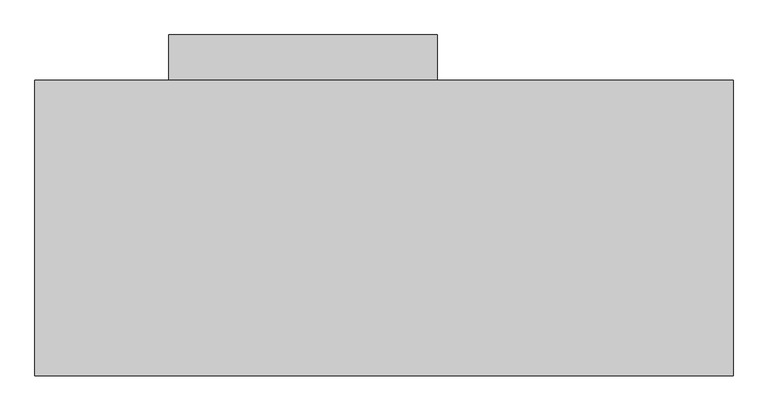
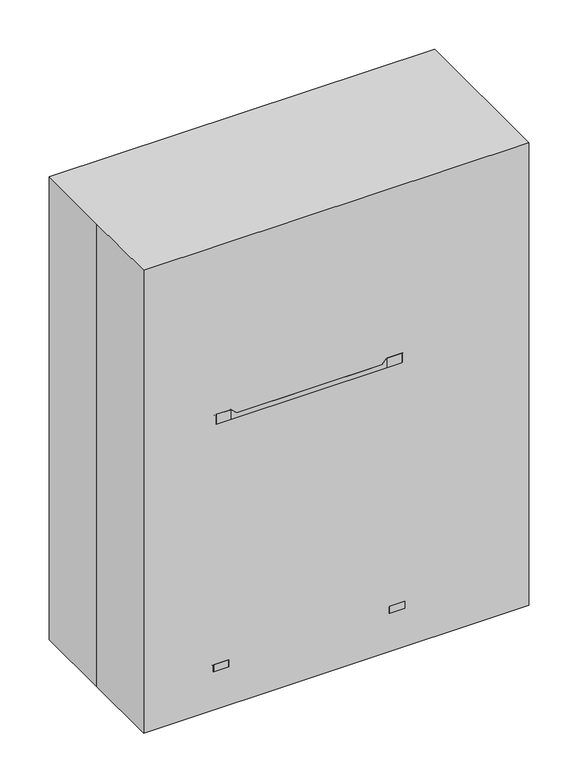
"""IFC4 building model written with IfcOpenShell, lengths in millimetres: proxy geometry, E0954 - Cart, Emergency, Mobile, 66H x 52W x 22D : E0954 - Cart, Emergency, Mobile, 66H x 52W x 22D."""

import ifcopenshell
import ifcopenshell.guid

model = None  # the IFC model being written
_history = None  # IfcOwnerHistory: only IFC2X3 demands one
_inside = {}  # id of a spatial element -> (the spatial element, [elements in it])
_under = {}  # id of a project, library or spatial element -> (it, [spatial elements below it])
_declared = {}  # id of a project -> (the project, [libraries it declares])
_typed = {}  # id of a type object -> (the type object, [elements of that type])
_made_of = {}  # id of a material, layer set ... -> (it, [elements and type objects made of it])


def new_model(schema):
    """Start an empty IFC model of exactly this schema.

    Asked for "IFC4X3", IfcOpenShell would pick the latest addendum, in which some entities
    have other attributes; the version numbers below select the first issue.
    IFC2X3 requires an IfcOwnerHistory on every rooted entity: one is made here for all.
    """
    global model, _history
    if schema == "IFC4X3":
        model = ifcopenshell.file(schema_version=(4, 3, 0, 0))
    else:
        model = ifcopenshell.file(schema=schema)
    _inside.clear()
    _under.clear()
    _declared.clear()
    _typed.clear()
    _made_of.clear()
    _history = None
    if model.schema == "IFC2X3":
        org = make("IfcOrganization", Name="unknown")
        user = make(
            "IfcPersonAndOrganization",
            ThePerson=make("IfcPerson", FamilyName="unknown"),
            TheOrganization=org,
        )
        app = make(
            "IfcApplication",
            ApplicationDeveloper=org,
            Version="unknown",
            ApplicationFullName="unknown",
            ApplicationIdentifier="unknown",
        )
        _history = make(
            "IfcOwnerHistory",
            OwningUser=user,
            OwningApplication=app,
            ChangeAction="ADDED",
            CreationDate=0,
        )
    return model


def make(cls, **values):
    """One entity of the class cls with the attributes given. An attribute that is None is left unset."""
    return model.create_entity(
        cls, **{name: value for name, value in values.items() if value is not None}
    )


def rooted(cls, **values):
    """An entity with a GlobalId (a new one), such as an element, a storey or a relation."""
    return make(cls, GlobalId=ifcopenshell.guid.new(), OwnerHistory=_history, **values)


def si_unit(unit_type, name, prefix=None):
    """IfcSIUnit, for example si_unit("LENGTHUNIT", "METRE", prefix="MILLI")."""
    return make("IfcSIUnit", UnitType=unit_type, Prefix=prefix, Name=name)


def assignment(units):
    """IfcUnitAssignment: the units of a project."""
    return None if units is None else make("IfcUnitAssignment", Units=units)


def point(xyz):
    """IfcCartesianPoint."""
    return None if xyz is None else make("IfcCartesianPoint", Coordinates=xyz)


def direction(xyz):
    """IfcDirection."""
    return None if xyz is None else make("IfcDirection", DirectionRatios=xyz)


def frame(location, z_axis=None, x_axis=None):
    """IfcAxis2Placement3D, a coordinate frame: its origin and axes. An axis left out is left unset."""
    return make(
        "IfcAxis2Placement3D",
        Location=point(location),
        Axis=direction(z_axis),
        RefDirection=direction(x_axis),
    )


def frame_2d(location, x_axis=None):
    """IfcAxis2Placement2D, a coordinate frame in the plane: its origin and x axis."""
    return make(
        "IfcAxis2Placement2D", Location=point(location), RefDirection=direction(x_axis)
    )


def origin():
    """The frame at (0, 0, 0) with its axes left unset."""
    return frame((0.0, 0.0, 0.0))


def origin_with_axes():
    """The frame at (0, 0, 0) with the z axis (0, 0, 1) and the x axis (1, 0, 0) written out."""
    return frame((0.0, 0.0, 0.0), z_axis=(0.0, 0.0, 1.0), x_axis=(1.0, 0.0, 0.0))


def place(relative_to, where):
    """IfcLocalPlacement: puts the frame where relative to a parent placement (None: the world)."""
    return make(
        "IfcLocalPlacement", PlacementRelTo=relative_to, RelativePlacement=where
    )


def context(
    kind, dimensions, precision=None, world=None, true_north=None, identifier=None
):
    """IfcGeometricRepresentationContext, for example the 3D "Model" context."""
    return make(
        "IfcGeometricRepresentationContext",
        ContextIdentifier=identifier,
        ContextType=kind,
        CoordinateSpaceDimension=dimensions,
        Precision=precision,
        WorldCoordinateSystem=world,
        TrueNorth=true_north,
    )


def project(units=None, contexts=None):
    """IfcProject with its units and contexts."""
    return rooted(
        "IfcProject",
        Name="project",
        RepresentationContexts=contexts,
        UnitsInContext=assignment(units),
    )


def spatial(cls, under=None, at=None, **own):
    """A site, building, storey or space (cls), placed at a placement, below another one or the project."""
    s = rooted(cls, ObjectPlacement=at, **own)
    if under is not None:
        _under.setdefault(under.id(), (under, []))[1].append(s)
    return s


def polyline(points):
    """IfcPolyline through the points."""
    return make("IfcPolyline", Points=[point(p) for p in points])


def circle_curve(where, radius):
    """IfcCircle in the frame where."""
    return make("IfcCircle", Position=where, Radius=radius)


def trimmed(basis, trim1, trim2, sense, master):
    """IfcTrimmedCurve: the piece of a basis curve between two trims."""
    return make(
        "IfcTrimmedCurve",
        BasisCurve=basis,
        Trim1=trim1,
        Trim2=trim2,
        SenseAgreement=sense,
        MasterRepresentation=master,
    )


def segment(curve, same_sense, transition):
    """IfcCompositeCurveSegment."""
    return make(
        "IfcCompositeCurveSegment",
        Transition=transition,
        SameSense=same_sense,
        ParentCurve=curve,
    )


def composite_curve(segments, self_intersect=None):
    """IfcCompositeCurve: segments joined end to end."""
    return make("IfcCompositeCurve", Segments=segments, SelfIntersect=self_intersect)


def outline(outer, holes=None, kind="AREA"):
    """IfcArbitraryClosedProfileDef: a profile drawn as a closed curve; with holes, ...WithVoids."""
    if holes is None:
        return make("IfcArbitraryClosedProfileDef", ProfileType=kind, OuterCurve=outer)
    return make(
        "IfcArbitraryProfileDefWithVoids",
        ProfileType=kind,
        OuterCurve=outer,
        InnerCurves=holes,
    )


def extrude(swept, where, along, depth):
    """IfcExtrudedAreaSolid: the profile swept, set in the frame where, extruded along a direction by depth."""
    return make(
        "IfcExtrudedAreaSolid",
        SweptArea=swept,
        Position=where,
        ExtrudedDirection=direction(along),
        Depth=depth,
    )


def faces_of(points, faces, orient=None, outer=None):
    """IfcFace entities. A face is a list of loops; a loop is a list of indices into points, from 0.

    orient and outer hold one flag for each loop. By default every Orientation is true, the
    first loop of a face is its IfcFaceOuterBound and the others are IfcFaceBound.
    """
    made = []
    for i, loops in enumerate(faces):
        bounds = []
        for j, loop in enumerate(loops):
            is_outer = j == 0 if outer is None else outer[i][j]
            bounds.append(
                make(
                    "IfcFaceOuterBound" if is_outer else "IfcFaceBound",
                    Bound=make("IfcPolyLoop", Polygon=[points[k] for k in loop]),
                    Orientation=True if orient is None else orient[i][j],
                )
            )
        made.append(make("IfcFace", Bounds=bounds))
    return made


def faceted_brep(points, faces, orient=None, outer=None, voids=None):
    """IfcFacetedBrep: a solid bounded by flat faces; with voids (closed shells), ...WithVoids."""
    shared = [point(p) for p in points]
    hull = make("IfcClosedShell", CfsFaces=faces_of(shared, faces, orient, outer))
    if voids is None:
        return make("IfcFacetedBrep", Outer=hull)
    return make(
        "IfcFacetedBrepWithVoids",
        Outer=hull,
        Voids=[
            make(cls, CfsFaces=faces_of(shared, fs, o, b)) for cls, fs, o, b in voids
        ],
    )


def shape(context_of_items, identifier, shape_type, items):
    """IfcShapeRepresentation: the items that make up one representation, for example the "Body"."""
    return make(
        "IfcShapeRepresentation",
        ContextOfItems=context_of_items,
        RepresentationIdentifier=identifier,
        RepresentationType=shape_type,
        Items=items,
    )


def source(mapping_origin, context_of_items, identifier, shape_type, items):
    """IfcRepresentationMap: a shape defined once, which mapped items show again and again."""
    return make(
        "IfcRepresentationMap",
        MappingOrigin=mapping_origin,
        MappedRepresentation=shape(context_of_items, identifier, shape_type, items),
    )


def transform(
    local_origin,
    x_axis=None,
    y_axis=None,
    z_axis=None,
    scale=None,
    scale2=None,
    scale3=None,
    uniform=True,
):
    """IfcCartesianTransformationOperator3D, or its non-uniform kind. x_axis, y_axis, z_axis: its Axis1, 2, 3."""
    if uniform:
        return make(
            "IfcCartesianTransformationOperator3D",
            Axis1=direction(x_axis),
            Axis2=direction(y_axis),
            LocalOrigin=point(local_origin),
            Scale=scale,
            Axis3=direction(z_axis),
        )
    return make(
        "IfcCartesianTransformationOperator3DnonUniform",
        Axis1=direction(x_axis),
        Axis2=direction(y_axis),
        LocalOrigin=point(local_origin),
        Scale=scale,
        Axis3=direction(z_axis),
        Scale2=scale2,
        Scale3=scale3,
    )


def mapped(mapping_source, mapping_target):
    """IfcMappedItem: shows the shape of a source again, moved by a transform."""
    return make(
        "IfcMappedItem", MappingSource=mapping_source, MappingTarget=mapping_target
    )


def made_of(thing, what):
    """Note that an element or type object is made of a material, layer set ...; save() writes the relation."""
    if what is not None:
        _made_of.setdefault(what.id(), (what, []))[1].append(thing)
    return thing


def element(
    cls,
    number,
    at=None,
    inside=None,
    cuts=None,
    type_object=None,
    material=None,
    context=None,
    identifier="Body",
    shape_type=None,
    held_by="IfcProductDefinitionShape",
    body=None,
    shapes=None,
    **own,
):
    """One element of the class cls, such as IfcWall. Its Tag is "e" and its number.

    at: its placement. inside: the storey or other place that contains it. cuts: it is an
    opening in that element (IfcRelVoidsElement). A single representation is given by context,
    identifier, shape_type and body (its items); several are given by shapes. held_by: the class
    of the entity that holds the representations. save() writes the other relations.
    """
    e = rooted(cls, Tag="e%d" % number, ObjectPlacement=at, **own)
    if body is not None:
        shapes = [shape(context, identifier, shape_type, body)]
    if shapes is not None:
        e.Representation = make(held_by, Representations=shapes)
    if inside is not None:
        _inside.setdefault(inside.id(), (inside, []))[1].append(e)
    if cuts is not None:
        rooted(
            "IfcRelVoidsElement", RelatingBuildingElement=cuts, RelatedOpeningElement=e
        )
    if type_object is not None:
        _typed.setdefault(type_object.id(), (type_object, []))[1].append(e)
    return made_of(e, material)


def aggregate(whole, parts):
    """IfcRelAggregates: a whole, such as a stair, and the parts it consists of."""
    return rooted("IfcRelAggregates", RelatingObject=whole, RelatedObjects=parts)


def save(model, path):
    """Write the relations noted so far, then the file.

    IfcRelAggregates (storeys below a building ...), IfcRelContainedInSpatialStructure (elements
    in a storey), IfcRelDefinesByType, IfcRelAssociatesMaterial and IfcRelDeclares: one each for
    every whole, place, type object, material and project.
    """
    for whole, parts in _under.values():
        aggregate(whole, parts)
    for where, things in _inside.values():
        rooted(
            "IfcRelContainedInSpatialStructure",
            RelatedElements=things,
            RelatingStructure=where,
        )
    for kind, things in _typed.values():
        rooted("IfcRelDefinesByType", RelatedObjects=things, RelatingType=kind)
    for what, things in _made_of.values():
        rooted("IfcRelAssociatesMaterial", RelatedObjects=things, RelatingMaterial=what)
    for by, libraries in _declared.values():
        rooted("IfcRelDeclares", RelatingContext=by, RelatedDefinitions=libraries)
    model.write(path)


def plane_surface(at):
    """IfcPlane: the flat surface through the origin of the frame at, square to its z axis."""
    return make("IfcPlane", Position=at)


def cylinder_surface(at, radius):
    """IfcCylindricalSurface: all points at the distance radius from the z axis of the frame at."""
    return make("IfcCylindricalSurface", Position=at, Radius=radius)


def revolved_surface(curve, axis_point, axis_direction):
    """IfcSurfaceOfRevolution: the curve turned about the line through axis_point along axis_direction."""
    return make(
        "IfcSurfaceOfRevolution",
        SweptCurve=make("IfcArbitraryOpenProfileDef", ProfileType="CURVE", Curve=curve),
        AxisPosition=make("IfcAxis1Placement", Location=point(axis_point), Axis=direction(axis_direction)),
    )


def spline_surface(u_degree, v_degree, points, u_multiplicities, v_multiplicities, u_knots, v_knots, weights=None):
    """IfcBSplineSurfaceWithKnots; with weights, IfcRationalBSplineSurfaceWithKnots. points: one row for each step in u."""
    own = dict(
        UDegree=u_degree,
        VDegree=v_degree,
        ControlPointsList=[[point(p) for p in row] for row in points],
        SurfaceForm="UNSPECIFIED",
        UClosed=False,
        VClosed=False,
        SelfIntersect=False,
        UMultiplicities=u_multiplicities,
        VMultiplicities=v_multiplicities,
        UKnots=u_knots,
        VKnots=v_knots,
        KnotSpec="UNSPECIFIED",
    )
    if weights is None:
        return make("IfcBSplineSurfaceWithKnots", **own)
    return make("IfcRationalBSplineSurfaceWithKnots", WeightsData=weights, **own)


def advanced_brep(points, edges, surfaces, faces):
    """IfcAdvancedBrep: a solid bounded by faces that lie on surfaces and meet in shared edges.

    An edge is (start, end): straight between two places in points (the first is 0);
    or (start, end, curve); or (start, end, curve, False) where it runs against its curve.
    A face is (place in surfaces, loops), or (place, loops, False) where it looks against
    its surface's normal. A loop lists edges by number (the first is 1), with a minus sign
    where the edge is run from its end to its start. The first loop is the outer one.
    """
    corners = [point(p) for p in points]
    vertices = [make("IfcVertexPoint", VertexGeometry=c) for c in corners]
    made = []
    for start, end, *more in edges:
        made.append(
            make(
                "IfcEdgeCurve",
                EdgeStart=vertices[start],
                EdgeEnd=vertices[end],
                EdgeGeometry=more[0] if more else make("IfcPolyline", Points=[corners[start], corners[end]]),
                SameSense=more[1] if len(more) > 1 else True,
            )
        )
    hull = []
    for where, loops, *sense in faces:
        bounds = []
        for j, loop in enumerate(loops):
            ring = [make("IfcOrientedEdge", EdgeElement=made[abs(k) - 1], Orientation=k > 0) for k in loop]
            bounds.append(
                make(
                    "IfcFaceOuterBound" if j == 0 else "IfcFaceBound",
                    Bound=make("IfcEdgeLoop", EdgeList=ring),
                    Orientation=True,
                )
            )
        hull.append(make("IfcAdvancedFace", Bounds=bounds, FaceSurface=surfaces[where], SameSense=sense[0] if sense else True))
    return make("IfcAdvancedBrep", Outer=make("IfcClosedShell", CfsFaces=hull))


def specialty_equipment_8fa30587(model_context):
    return source(origin(), model_context, "Body", "SolidModel", [
        advanced_brep(
        [(-617.6487952, 2.9144028, 860.7975437), (-414.4487952, 2.9144028, 860.7975437), (-604.9487952, 2.9144028, 860.7975437), (-427.1487952, 2.9144028, 860.7975437), (-617.6487952, 2.9144028, 234.3936643), (-414.4487952, 2.9144028, 234.3936643), (-604.9487952, 2.9144028, 234.3936643), (-427.1487952, 2.9144028, 234.3936643), (-617.6487952, 2.9144028, 845.5698121), (-424.9008141, -41.9699547, 845.5698121), (-424.9008141, -41.9699547, 567.7573121), (-617.6487952, 2.9144028, 567.7573121), (-609.0105353, -38.0816322, 262.9573121), (-609.0105353, -38.0816322, 548.7073121), (-422.9407954, -37.7483612, 548.7073121), (-422.9407954, -37.7483612, 262.9573121), (-424.9008141, 47.7987602, 567.7573121), (-424.9008141, 47.7987602, 845.5698121), (-609.0105353, 43.9104377, 548.7073121), (-609.0105353, 43.9104377, 262.9573121), (-422.9407954, 43.5771667, 262.9573121), (-422.9407954, 43.5771667, 548.7073121), (-604.9487952, 2.9144028, 845.5698121), (-427.1487952, 2.9144028, 845.5698121), (-427.1487952, 2.9144028, 262.9573121), (-604.9487952, 2.9144028, 262.9573121), (-427.1487952, 2.9144028, 567.7573121), (-604.9487952, 2.9144028, 567.7573121), (-604.9487952, 2.9144028, 548.7073121), (-427.1487952, 2.9144028, 548.7073121)],
        [
            (0, 1, circle_curve(frame((-516.0487952, 2.9144028, 860.7975437), z_axis=(0.0, 0.0, 1.0), x_axis=(1.0, 1.2023715356688048e-12, 0.0)), 101.6)),
            (1, 0, circle_curve(frame((-516.0487952, 2.9144028, 860.7975437), z_axis=(0.0, 0.0, 1.0), x_axis=(1.0, 1.2023715356688048e-12, 0.0)), 101.6)),
            (2, 3, circle_curve(frame((-516.0487952, 2.9144028, 860.7975437), z_axis=(0.0, 0.0, -1.0), x_axis=(1.0, 1.2023715356688048e-12, 0.0)), 88.9)),
            (3, 2, circle_curve(frame((-516.0487952, 2.9144028, 860.7975437), z_axis=(0.0, 0.0, -1.0), x_axis=(1.0, 1.2023715356688048e-12, 0.0)), 88.9)),
            (4, 5, circle_curve(frame((-516.0487952, 2.9144028, 234.3936643), z_axis=(0.0, 0.0, -1.0), x_axis=(1.0, 1.2023715356688048e-12, 0.0)), 101.6)),
            (5, 4, circle_curve(frame((-516.0487952, 2.9144028, 234.3936643), z_axis=(0.0, 0.0, -1.0), x_axis=(1.0, 1.2023715356688048e-12, 0.0)), 101.6)),
            (6, 7, circle_curve(frame((-516.0487952, 2.9144028, 234.3936643), z_axis=(0.0, 0.0, 1.0), x_axis=(1.0, 1.2023715356688048e-12, 0.0)), 88.9)),
            (7, 6, circle_curve(frame((-516.0487952, 2.9144028, 234.3936643), z_axis=(0.0, 0.0, 1.0), x_axis=(1.0, 1.2023715356688048e-12, 0.0)), 88.9)),
            (0, 8),
            (8, 9, circle_curve(frame((-516.0487952, 2.9144028, 845.5698121), z_axis=(0.0, 0.0, 1.0), x_axis=(1.0, 1.2023715356688048e-12, 0.0)), 101.6)),
            (9, 10),
            (10, 11, circle_curve(frame((-516.0487952, 2.9144028, 567.7573121), z_axis=(0.0, 0.0, -1.0), x_axis=(1.0, 1.2023715356688048e-12, 0.0)), 101.6)),
            (11, 4),
            (5, 1),
            (12, 13),
            (13, 14, circle_curve(frame((-516.0487952, 2.9144028, 548.7073121), z_axis=(0.0, 0.0, 1.0), x_axis=(1.0, 1.2023715356688048e-12, 0.0)), 101.6)),
            (14, 15),
            (15, 12, circle_curve(frame((-516.0487952, 2.9144028, 262.9573121), z_axis=(0.0, 0.0, -1.0), x_axis=(1.0, 1.2023715356688048e-12, 0.0)), 101.6)),
            (11, 16, circle_curve(frame((-516.0487952, 2.9144028, 567.7573121), z_axis=(0.0, 0.0, -1.0), x_axis=(1.0, 1.2023715356688048e-12, 0.0)), 101.6)),
            (16, 17),
            (17, 8, circle_curve(frame((-516.0487952, 2.9144028, 845.5698121), z_axis=(0.0, 0.0, 1.0), x_axis=(1.0, 1.2023715356688048e-12, 0.0)), 101.6)),
            (18, 19),
            (19, 20, circle_curve(frame((-516.0487952, 2.9144028, 262.9573121), z_axis=(0.0, 0.0, -1.0), x_axis=(1.0, 1.2023715356688048e-12, 0.0)), 101.6)),
            (20, 21),
            (21, 18, circle_curve(frame((-516.0487952, 2.9144028, 548.7073121), z_axis=(0.0, 0.0, 1.0), x_axis=(1.0, 1.2023715356688048e-12, 0.0)), 101.6)),
            (2, 22),
            (22, 23, circle_curve(frame((-516.0487952, 2.9144028, 845.5698121), z_axis=(0.0, 0.0, -1.0), x_axis=(1.0, 1.2023715356688048e-12, 0.0)), 88.9)),
            (23, 3),
            (7, 24),
            (24, 25, circle_curve(frame((-516.0487952, 2.9144028, 262.9573121), z_axis=(0.0, 0.0, 1.0), x_axis=(1.0, 1.2023715356688048e-12, 0.0)), 88.9)),
            (25, 6),
            (26, 27, circle_curve(frame((-516.0487952, 2.9144028, 567.7573121), z_axis=(0.0, 0.0, 1.0), x_axis=(1.0, 1.2023715356688048e-12, 0.0)), 88.9)),
            (27, 28),
            (28, 29, circle_curve(frame((-516.0487952, 2.9144028, 548.7073121), z_axis=(0.0, 0.0, -1.0), x_axis=(1.0, 1.2023715356688048e-12, 0.0)), 88.9)),
            (29, 26),
            (23, 22, circle_curve(frame((-516.0487952, 2.9144028, 845.5698121), z_axis=(0.0, 0.0, -1.0), x_axis=(1.0, 1.2023715356688048e-12, 0.0)), 88.9)),
            (25, 24, circle_curve(frame((-516.0487952, 2.9144028, 262.9573121), z_axis=(0.0, 0.0, 1.0), x_axis=(1.0, 1.2023715356688048e-12, 0.0)), 88.9)),
            (27, 26, circle_curve(frame((-516.0487952, 2.9144028, 567.7573121), z_axis=(0.0, 0.0, 1.0), x_axis=(1.0, 1.2023715356688048e-12, 0.0)), 88.9)),
            (29, 28, circle_curve(frame((-516.0487952, 2.9144028, 548.7073121), z_axis=(0.0, 0.0, -1.0), x_axis=(1.0, 1.2023715356688048e-12, 0.0)), 88.9)),
            (10, 16),
            (9, 17),
            (18, 13),
            (12, 19),
            (15, 20),
            (14, 21),
        ],
        [
            plane_surface(frame((-414.4487952, 2.9144028, 860.7975437), z_axis=(0.0, 0.0, 1.0), x_axis=(-1.2023715356688048e-12, 1.0, 0.0))),
            plane_surface(frame((-414.4487952, 2.9144028, 234.3936643), z_axis=(0.0, 0.0, -1.0), x_axis=(1.2023715356688048e-12, -1.0, 0.0))),
            cylinder_surface(frame((-516.0487952, 2.9144028, 234.3936643), z_axis=(0.0, 0.0, 1.0), x_axis=(1.0, 1.2023715356688048e-12, 0.0)), 101.6),
            revolved_surface(polyline([(-427.1487952, 2.914402800106891, 845.5698121), (-427.1487952, 2.914402800106891, 860.7975437)]), (-516.0487952, 2.9144028, 163.5125), (0.0, 0.0, -1.0)),
            revolved_surface(polyline([(-427.1487952, 2.914402800106891, 234.3936643), (-427.1487952, 2.914402800106891, 262.9573121)]), (-516.0487952, 2.9144028, 163.5125), (0.0, 0.0, -1.0)),
            revolved_surface(polyline([(-427.1487952, 2.914402800106891, 548.7073121), (-427.1487952, 2.914402800106891, 567.7573121)]), (-516.0487952, 2.9144028, 163.5125), (0.0, 0.0, -1.0)),
            plane_surface(frame((-628.0605353, -110.1467187, 567.7573121), z_axis=(0.0, 0.0, 1.0), x_axis=(0.0, 1.0, 0.0))),
            plane_surface(frame((-424.9008141, -110.1467187, 567.7573121), z_axis=(-1.0, 0.0, 0.0), x_axis=(0.0, 1.0, 0.0))),
            plane_surface(frame((-424.9008141, -110.1467187, 845.5698121), z_axis=(0.0, 0.0, -1.0), x_axis=(0.0, 1.0, 0.0))),
            plane_surface(frame((-609.0105353, -110.1467187, 548.7073121), z_axis=(1.0, 0.0, 0.0), x_axis=(0.0, 1.0, 0.0))),
            plane_surface(frame((-609.0105353, -110.1467187, 262.9573121), z_axis=(0.0, 0.0, 1.0), x_axis=(0.0, 1.0, 0.0))),
            plane_surface(frame((-422.9407954, -110.1467187, 262.9573121), z_axis=(-1.0, 0.0, 0.0), x_axis=(0.0, 1.0, 0.0))),
            plane_surface(frame((-422.9407954, -110.1467187, 548.7073121), z_axis=(0.0, 0.0, -1.0), x_axis=(0.0, 1.0, 0.0))),
        ],
        [
            (0, [[1, 2], [3, 4]]),
            (1, [[5, 6], [7, 8]]),
            (2, [[-1, 9, 10, 11, 12, 13, -6, 14], [15, 16, 17, 18]]),
            (2, [[-2, -14, -5, -13, 19, 20, 21, -9], [22, 23, 24, 25]]),
            (3, [[-3, 26, 27, 28]]),
            (4, [[-8, 29, 30, 31]]),
            (5, [[32, 33, 34, 35]]),
            (3, [[-4, -28, 36, -26]]),
            (4, [[-7, -31, 37, -29]]),
            (5, [[38, -35, 39, -33]]),
            (6, [[40, -19, -12], [-32, -38]]),
            (7, [[-40, -11, 41, -20]]),
            (8, [[-41, -10, -21], [-27, -36]]),
            (9, [[42, -15, 43, -22]]),
            (10, [[-43, -18, 44, -23], [-30, -37]]),
            (11, [[-44, -17, 45, -24]]),
            (12, [[-42, -25, -45, -16], [-34, -39]]),
        ],
    ),
        faceted_brep([(224.7592046, -250.6571972, 163.5125), (224.7592046, -250.6571972, 1031.748), (173.9592046, -250.6571972, 1031.748), (-359.4407954, -250.6571972, 1031.748), (-410.2407954, -250.6571972, 1031.748), (-410.2407954, -250.6571972, 163.5125), (-359.4407954, -250.6571972, 221.742), (-359.4407954, -250.6571972, 996.442), (173.9592046, -250.6571972, 996.442), (173.9592046, -250.6571972, 221.742), (224.7592046, 250.9928028, 163.5125), (-410.2407954, 250.9928028, 163.5125), (-410.2407954, 250.9928028, 1031.748), (-359.4407954, 250.9928028, 1031.748), (173.9592046, 250.9928028, 1031.748), (224.7592046, 250.9928028, 1031.748), (-359.4407954, 238.7231785, 996.442), (-359.4407954, 238.7231785, 221.742), (173.9592046, 238.7231785, 221.742), (173.9592046, 238.7231785, 996.442)], [[[0, 1, 2, 3, 4, 5], [6, 7, 8, 9]], [[10, 11, 12, 13, 14, 15]], [[1, 0, 10, 15]], [[2, 1, 15, 14]], [[3, 2, 14, 13]], [[4, 3, 13, 12]], [[5, 4, 12, 11]], [[0, 5, 11, 10]], [[16, 17, 18, 19]], [[17, 16, 7, 6]], [[18, 17, 6, 9]], [[19, 18, 9, 8]], [[16, 19, 8, 7]]]),
        extrude(outline(polyline([(154.9092046, 154.1553028), (154.9092046, -204.6196972), (-340.3907954, -204.6196972), (-340.3907954, 154.1553028), (154.9092046, 154.1553028)])), frame((0.0, 0.0, 912.2918), z_axis=(0.0, 0.0, 1.0), x_axis=(1.0, 0.0, 0.0)), (0.0, 0.0, 1.0), 76.4986177),
        extrude(outline(polyline([(154.9092046, 154.1553028), (154.9092046, -204.6196972), (-340.3907954, -204.6196972), (-340.3907954, 154.1553028), (154.9092046, 154.1553028)])), frame((0.0, 0.0, 835.7931823), z_axis=(0.0, 0.0, 1.0), x_axis=(1.0, 0.0, 0.0)), (0.0, 0.0, 1.0), 76.4986177),
        extrude(outline(polyline([(154.9092046, 154.1553028), (154.9092046, -204.6196972), (-340.3907954, -204.6196972), (-340.3907954, 154.1553028), (154.9092046, 154.1553028)])), frame((0.0, 0.0, 759.4438734), z_axis=(0.0, 0.0, 1.0), x_axis=(1.0, 0.0, 0.0)), (0.0, 0.0, 1.0), 76.4986177),
        extrude(outline(polyline([(154.9092046, 154.1553028), (154.9092046, -204.6196972), (-340.3907954, -204.6196972), (-340.3907954, 154.1553028), (154.9092046, 154.1553028)])), frame((0.0, 0.0, 683.0945645), z_axis=(0.0, 0.0, 1.0), x_axis=(1.0, 0.0, 0.0)), (0.0, 0.0, 1.0), 76.4986177),
        extrude(outline(polyline([(154.9092046, 154.1553028), (154.9092046, -204.6196972), (-340.3907954, -204.6196972), (-340.3907954, 154.1553028), (154.9092046, 154.1553028)])), frame((0.0, 0.0, 530.3959468), z_axis=(0.0, 0.0, 1.0), x_axis=(1.0, 0.0, 0.0)), (0.0, 0.0, 1.0), 152.6986177),
        extrude(outline(polyline([(154.9092046, 154.1553028), (154.9092046, -204.6196972), (-340.3907954, -204.6196972), (-340.3907954, 154.1553028), (154.9092046, 154.1553028)])), frame((0.0, 0.0, 377.6973291), z_axis=(0.0, 0.0, 1.0), x_axis=(1.0, 0.0, 0.0)), (0.0, 0.0, 1.0), 152.6986177),
        extrude(outline(polyline([(154.9092046, 154.1553028), (154.9092046, -204.6196972), (-340.3907954, -204.6196972), (-340.3907954, 154.1553028), (154.9092046, 154.1553028)])), frame((0.0, 0.0, 225.2973291), z_axis=(0.0, 0.0, 1.0), x_axis=(1.0, 0.0, 0.0)), (0.0, 0.0, 1.0), 152.4),
        extrude(outline(composite_curve([segment(polyline([(1576.3284075, 82.0502646), (1573.7217185, 79.4435756)]), True, "CONTINUOUS"), segment(trimmed(circle_curve(frame_2d((1564.938779, 70.6606361)), 12.4209521), [point((1573.7217185, 79.4435756))], [point((1577.3597311, 70.6606361))], True, "CARTESIAN"), True, "CONTINUOUS"), segment(polyline([(1577.3597311, 70.6606361), (1577.3597311, 297.5600485)]), True, "CONTINUOUS"), segment(trimmed(circle_curve(frame_2d((1564.938779, 297.5600485)), 12.4209521), [point((1577.3597311, 297.5600485))], [point((1573.7217185, 288.777109))], True, "CARTESIAN"), True, "CONTINUOUS"), segment(polyline([(1573.7217185, 288.777109), (1576.3284075, 286.17042)]), True, "CONTINUOUS"), segment(trimmed(circle_curve(frame_2d((1564.938779, 297.5600485)), 16.1073671), [point((1576.3284075, 286.17042))], [point((1581.0461461, 297.5600485))], False, "CARTESIAN"), True, "CONTINUOUS"), segment(polyline([(1581.0461461, 297.5600485), (1581.0461461, 70.6606361)]), True, "CONTINUOUS"), segment(trimmed(circle_curve(frame_2d((1564.938779, 70.6606361)), 16.1073671), [point((1581.0461461, 70.6606361))], [point((1576.3284075, 82.0502646))], False, "CARTESIAN"), True, "CONTINUOUS")], self_intersect=False)), frame((0.0, 172.0713619, 0.0), z_axis=(0.0, 1.0, 0.0), x_axis=(0.0, 0.0, 1.0)), (0.0, 0.0, 1.0), 3.1474566),
        extrude(outline(composite_curve([segment(trimmed(circle_curve(frame_2d((183.4842046, 174.7928028)), 12.7), [point((183.4842046, 187.4928028))], [point((183.4842046, 162.0928028))], False, "CARTESIAN"), True, "CONTINUOUS"), segment(trimmed(circle_curve(frame_2d((183.4842046, 174.7928028)), 12.7), [point((183.4842046, 162.0928028))], [point((183.4842046, 187.4928028))], False, "CARTESIAN"), True, "CONTINUOUS")], self_intersect=False)), frame((0.0, 0.0, 1031.748), z_axis=(0.0, 0.0, 1.0), x_axis=(1.0, 0.0, 0.0)), (0.0, 0.0, 1.0), 558.8),
        extrude(outline(polyline([(46.9592046, 333.5428028), (46.9592046, 263.6928028), (161.2592046, 263.6928028), (161.2592046, 250.9928028), (-346.7407954, 250.9928028), (-346.7407954, 263.6928028), (-232.4407954, 263.6928028), (-232.4407954, 333.5428028), (46.9592046, 333.5428028)])), frame((0.0, 0.0, 759.5931823), z_axis=(0.0, 0.0, 1.0), x_axis=(1.0, 0.0, 0.0)), (0.0, 0.0, 1.0), 51.55692),
        extrude(outline(composite_curve([segment(polyline([(-368.9657954, -279.2321972), (-419.7657954, -279.2321972)]), True, "CONTINUOUS"), segment(trimmed(circle_curve(frame_2d((-419.7657954, -253.8321972)), 25.4), [point((-419.7657954, -279.2321972))], [point((-445.1657954, -253.8321972))], False, "CARTESIAN"), True, "CONTINUOUS"), segment(polyline([(-445.1657954, -253.8321972), (-445.1657954, -203.0321972)]), True, "CONTINUOUS"), segment(trimmed(circle_curve(frame_2d((-419.7657954, -203.0321972)), 25.4), [point((-445.1657954, -203.0321972))], [point((-419.7657954, -177.6321972))], False, "CARTESIAN"), True, "CONTINUOUS"), segment(polyline([(-419.7657954, -177.6321972), (-368.9657954, -177.6321972)]), True, "CONTINUOUS"), segment(trimmed(circle_curve(frame_2d((-368.9657954, -203.0321972)), 25.4), [point((-368.9657954, -177.6321972))], [point((-343.5657954, -203.0321972))], False, "CARTESIAN"), True, "CONTINUOUS"), segment(polyline([(-343.5657954, -203.0321972), (-343.5657954, -253.8321972)]), True, "CONTINUOUS"), segment(trimmed(circle_curve(frame_2d((-368.9657954, -253.8321972)), 25.4), [point((-343.5657954, -253.8321972))], [point((-368.9657954, -279.2321972))], False, "CARTESIAN"), True, "CONTINUOUS")], self_intersect=False)), frame((0.0, 0.0, 138.1125), z_axis=(0.0, 0.0, 1.0), x_axis=(1.0, 0.0, 0.0)), (0.0, 0.0, 1.0), 25.4),
        extrude(outline(composite_curve([segment(trimmed(circle_curve(frame_2d((183.4842046, -253.8321972)), 25.4), [point((183.4842046, -279.2321972))], [point((158.0842046, -253.8321972))], False, "CARTESIAN"), True, "CONTINUOUS"), segment(polyline([(158.0842046, -253.8321972), (158.0842046, -203.0321972)]), True, "CONTINUOUS"), segment(trimmed(circle_curve(frame_2d((183.4842046, -203.0321972)), 25.4), [point((158.0842046, -203.0321972))], [point((183.4842046, -177.6321972))], False, "CARTESIAN"), True, "CONTINUOUS"), segment(polyline([(183.4842046, -177.6321972), (234.2842046, -177.6321972)]), True, "CONTINUOUS"), segment(trimmed(circle_curve(frame_2d((234.2842046, -203.0321972)), 25.4), [point((234.2842046, -177.6321972))], [point((259.6842046, -203.0321972))], False, "CARTESIAN"), True, "CONTINUOUS"), segment(polyline([(259.6842046, -203.0321972), (259.6842046, -253.8321972)]), True, "CONTINUOUS"), segment(trimmed(circle_curve(frame_2d((234.2842046, -253.8321972)), 25.4), [point((259.6842046, -253.8321972))], [point((234.2842046, -279.2321972))], False, "CARTESIAN"), True, "CONTINUOUS"), segment(polyline([(234.2842046, -279.2321972), (183.4842046, -279.2321972)]), True, "CONTINUOUS")], self_intersect=False)), frame((0.0, 0.0, 138.1125), z_axis=(0.0, 0.0, 1.0), x_axis=(1.0, 0.0, 0.0)), (0.0, 0.0, 1.0), 25.4),
        extrude(outline(composite_curve([segment(trimmed(circle_curve(frame_2d((-419.7657954, 254.1678028)), 25.4), [point((-445.1657954, 254.1678028))], [point((-419.7657954, 279.5678028))], False, "CARTESIAN"), True, "CONTINUOUS"), segment(polyline([(-419.7657954, 279.5678028), (-368.9657954, 279.5678028)]), True, "CONTINUOUS"), segment(trimmed(circle_curve(frame_2d((-368.9657954, 254.1678028)), 25.4), [point((-368.9657954, 279.5678028))], [point((-343.5657954, 254.1678028))], False, "CARTESIAN"), True, "CONTINUOUS"), segment(polyline([(-343.5657954, 254.1678028), (-343.5657954, 203.3678028)]), True, "CONTINUOUS"), segment(trimmed(circle_curve(frame_2d((-368.9657954, 203.3678028)), 25.4), [point((-343.5657954, 203.3678028))], [point((-368.9657954, 177.9678028))], False, "CARTESIAN"), True, "CONTINUOUS"), segment(polyline([(-368.9657954, 177.9678028), (-419.7657954, 177.9678028)]), True, "CONTINUOUS"), segment(trimmed(circle_curve(frame_2d((-419.7657954, 203.3678028)), 25.4), [point((-419.7657954, 177.9678028))], [point((-445.1657954, 203.3678028))], False, "CARTESIAN"), True, "CONTINUOUS"), segment(polyline([(-445.1657954, 203.3678028), (-445.1657954, 254.1678028)]), True, "CONTINUOUS")], self_intersect=False)), frame((0.0, 0.0, 138.1125), z_axis=(0.0, 0.0, 1.0), x_axis=(1.0, 0.0, 0.0)), (0.0, 0.0, 1.0), 25.4),
        extrude(outline(composite_curve([segment(trimmed(circle_curve(frame_2d((183.4842046, 254.1678028)), 25.4), [point((158.0842046, 254.1678028))], [point((183.4842046, 279.5678028))], False, "CARTESIAN"), True, "CONTINUOUS"), segment(polyline([(183.4842046, 279.5678028), (234.2842046, 279.5678028)]), True, "CONTINUOUS"), segment(trimmed(circle_curve(frame_2d((234.2842046, 254.1678028)), 25.4), [point((234.2842046, 279.5678028))], [point((259.6842046, 254.1678028))], False, "CARTESIAN"), True, "CONTINUOUS"), segment(polyline([(259.6842046, 254.1678028), (259.6842046, 203.3678028)]), True, "CONTINUOUS"), segment(trimmed(circle_curve(frame_2d((234.2842046, 203.3678028)), 25.4), [point((259.6842046, 203.3678028))], [point((234.2842046, 177.9678028))], False, "CARTESIAN"), True, "CONTINUOUS"), segment(polyline([(234.2842046, 177.9678028), (183.4842046, 177.9678028)]), True, "CONTINUOUS"), segment(trimmed(circle_curve(frame_2d((183.4842046, 203.3678028)), 25.4), [point((183.4842046, 177.9678028))], [point((158.0842046, 203.3678028))], False, "CARTESIAN"), True, "CONTINUOUS"), segment(polyline([(158.0842046, 203.3678028), (158.0842046, 254.1678028)]), True, "CONTINUOUS")], self_intersect=False)), frame((0.0, 0.0, 138.1125), z_axis=(0.0, 0.0, 1.0), x_axis=(1.0, 0.0, 0.0)), (0.0, 0.0, 1.0), 25.4),
        extrude(outline(composite_curve([segment(trimmed(circle_curve(frame_2d((60.3746094, -384.791186)), 60.3746094), [point((60.3746094, -324.4165766))], [point((60.3746094, -445.1657954))], False, "CARTESIAN"), True, "CONTINUOUS"), segment(trimmed(circle_curve(frame_2d((60.3746094, -384.791186)), 60.3746094), [point((60.3746094, -445.1657954))], [point((60.3746094, -324.4165766))], False, "CARTESIAN"), True, "CONTINUOUS")], self_intersect=False)), frame((0.0, 219.2428028, 0.0), z_axis=(0.0, 1.0, 0.0), x_axis=(0.0, 0.0, 1.0)), (0.0, 0.0, 1.0), 19.05),
        extrude(outline(composite_curve([segment(trimmed(circle_curve(frame_2d((60.3746094, 199.3095952)), 60.3746094), [point((60.3746094, 259.6842046))], [point((60.3746094, 138.9349859))], False, "CARTESIAN"), True, "CONTINUOUS"), segment(trimmed(circle_curve(frame_2d((60.3746094, 199.3095952)), 60.3746094), [point((60.3746094, 138.9349859))], [point((60.3746094, 259.6842046))], False, "CARTESIAN"), True, "CONTINUOUS")], self_intersect=False)), frame((0.0, 219.2428028, 0.0), z_axis=(0.0, 1.0, 0.0), x_axis=(0.0, 0.0, 1.0)), (0.0, 0.0, 1.0), 19.05),
        extrude(outline(polyline([(60.3746094, -391.141186), (60.3746094, -378.441186), (138.1125, -332.4532954), (138.1125, -445.1657954), (60.3746094, -391.141186)])), frame((0.0, 216.0678028, 0.0), z_axis=(0.0, 1.0, 0.0), x_axis=(0.0, 0.0, 1.0)), (0.0, 0.0, 1.0), 25.4),
        extrude(outline(polyline([(60.3746094, 192.9595952), (60.3746094, 205.6595952), (138.1125, 259.6842046), (138.1125, 146.9717046), (60.3746094, 192.9595952)])), frame((0.0, 216.0678028, 0.0), z_axis=(0.0, 1.0, 0.0), x_axis=(0.0, 0.0, 1.0)), (0.0, 0.0, 1.0), 25.4),
        extrude(outline(composite_curve([segment(trimmed(circle_curve(frame_2d((60.3746094, -384.791186)), 60.3746094), [point((60.3746094, -324.4165766))], [point((60.3746094, -445.1657954))], False, "CARTESIAN"), True, "CONTINUOUS"), segment(trimmed(circle_curve(frame_2d((60.3746094, -384.791186)), 60.3746094), [point((60.3746094, -445.1657954))], [point((60.3746094, -324.4165766))], False, "CARTESIAN"), True, "CONTINUOUS")], self_intersect=False)), frame((0.0, -237.9571972, 0.0), z_axis=(0.0, 1.0, 0.0), x_axis=(0.0, 0.0, 1.0)), (0.0, 0.0, 1.0), 19.05),
        extrude(outline(composite_curve([segment(trimmed(circle_curve(frame_2d((60.3746094, 199.3095952)), 60.3746094), [point((60.3746094, 259.6842046))], [point((60.3746094, 138.9349859))], False, "CARTESIAN"), True, "CONTINUOUS"), segment(trimmed(circle_curve(frame_2d((60.3746094, 199.3095952)), 60.3746094), [point((60.3746094, 138.9349859))], [point((60.3746094, 259.6842046))], False, "CARTESIAN"), True, "CONTINUOUS")], self_intersect=False)), frame((0.0, -237.9571972, 0.0), z_axis=(0.0, 1.0, 0.0), x_axis=(0.0, 0.0, 1.0)), (0.0, 0.0, 1.0), 19.05),
        extrude(outline(polyline([(60.3746094, -391.141186), (60.3746094, -378.441186), (138.1125, -332.4532954), (138.1125, -445.1657954), (60.3746094, -391.141186)])), frame((0.0, -241.1321972, 0.0), z_axis=(0.0, 1.0, 0.0), x_axis=(0.0, 0.0, 1.0)), (0.0, 0.0, 1.0), 25.4),
        extrude(outline(polyline([(60.3746094, 192.9595952), (60.3746094, 205.6595952), (138.1125, 259.6842046), (138.1125, 146.9717046), (60.3746094, 192.9595952)])), frame((0.0, -241.1321972, 0.0), z_axis=(0.0, 1.0, 0.0), x_axis=(0.0, 0.0, 1.0)), (0.0, 0.0, 1.0), 25.4),
        advanced_brep(
        [(434.3092046, -120.4821972, 590.55), (434.3092046, 120.8178028, 590.55), (408.9092046, 146.2178028, 590.55), (250.1592046, 146.2178028, 590.55), (224.7592046, 120.8178028, 590.55), (224.7592046, -120.4821972, 590.55), (250.1592046, -145.8821972, 590.55), (408.9092046, -145.8821972, 590.55), (408.9092046, -114.1321972, 273.05), (402.5592046, -120.4821972, 273.05), (256.5092046, -120.4821972, 273.05), (250.1592046, -114.1321972, 273.05), (250.1592046, 114.4678028, 273.05), (256.5092046, 120.8178028, 273.05), (402.5592046, 120.8178028, 273.05), (408.9092046, 114.4678028, 273.05)],
        [
            (0, 1),
            (1, 2, circle_curve(frame((408.9092046, 120.8178028, 590.55), z_axis=(0.0, 0.0, 1.0), x_axis=(0.0, -1.0, 0.0)), 25.4)),
            (2, 3),
            (3, 4, circle_curve(frame((250.1592046, 120.8178028, 590.55), z_axis=(0.0, 0.0, 1.0), x_axis=(0.0, -1.0, 0.0)), 25.4)),
            (4, 5),
            (5, 6, circle_curve(frame((250.1592046, -120.4821972, 590.55), z_axis=(0.0, 0.0, 1.0), x_axis=(0.0, -1.0, 0.0)), 25.4)),
            (6, 7),
            (7, 0, circle_curve(frame((408.9092046, -120.4821972, 590.55), z_axis=(0.0, 0.0, 1.0), x_axis=(0.0, -1.0, 0.0)), 25.4)),
            (8, 9, circle_curve(frame((402.5592046, -114.1321972, 273.05), z_axis=(0.0, 0.0, -1.0), x_axis=(0.0, -1.0, 0.0)), 6.35)),
            (9, 10),
            (10, 11, circle_curve(frame((256.5092046, -114.1321972, 273.05), z_axis=(0.0, 0.0, -1.0), x_axis=(0.0, -1.0, 0.0)), 6.35)),
            (11, 12),
            (12, 13, circle_curve(frame((256.5092046, 114.4678028, 273.05), z_axis=(0.0, 0.0, -1.0), x_axis=(0.0, -1.0, 0.0)), 6.35)),
            (13, 14),
            (14, 15, circle_curve(frame((402.5592046, 114.4678028, 273.05), z_axis=(0.0, 0.0, -1.0), x_axis=(0.0, -1.0, 0.0)), 6.35)),
            (15, 8),
            (15, 1),
            (0, 8),
            (14, 2),
            (13, 3),
            (12, 4),
            (11, 5),
            (10, 6),
            (9, 7),
        ],
        [
            plane_surface(frame((329.5342046, 0.1678028, 590.55), z_axis=(0.0, 0.0, 1.0), x_axis=(0.0, 1.0, 0.0))),
            plane_surface(frame((329.5342046, 0.1678028, 273.05), z_axis=(0.0, 0.0, -1.0), x_axis=(0.0, 1.0, 0.0))),
            plane_surface(frame((408.9092046, 0.1678028, 273.05), z_axis=(0.9968152785361276, 0.0, -0.07974522228285794), x_axis=(0.0, 1.0, 0.0))),
            spline_surface(2, 1, [[(408.9092046, 114.4678028, 273.05), (434.3092046, 120.8178028, 590.55)], [(408.9092046, 120.81780280000002, 273.05), (434.3092046, 146.21780279999996, 590.55)], [(402.5592046, 120.8178028, 273.05), (408.9092046, 146.2178028, 590.55)]], [3, 3], [2, 2], [0.0, 1.0], [0.0, 1.0], weights=[[1.0, 1.0], [0.7071067811865477, 0.7071067811865477], [1.0, 1.0]]),
            plane_surface(frame((329.5342046, 120.8178028, 273.05), z_axis=(0.0, 0.9968152785361256, -0.07974522228288214), x_axis=(-1.0, 0.0, 0.0))),
            spline_surface(2, 1, [[(256.5092046, 120.8178028, 273.05), (250.1592046, 146.2178028, 590.55)], [(250.15920459999998, 120.8178028, 273.05), (224.75920460000003, 146.21780279999996, 590.55)], [(250.1592046, 114.4678028, 273.05), (224.7592046, 120.8178028, 590.55)]], [3, 3], [2, 2], [0.0, 1.0], [0.0, 1.0], weights=[[1.0, 1.0], [0.7071067811865478, 0.7071067811865478], [1.0, 1.0]]),
            plane_surface(frame((250.1592046, 0.1678028, 273.05), z_axis=(-0.9968152785361235, 0.0, -0.07974522228290898), x_axis=(0.0, -1.0, 0.0))),
            spline_surface(2, 1, [[(250.1592046, -114.1321972, 273.05), (224.7592046, -120.4821972, 590.55)], [(250.1592046, -120.48219719999996, 273.05), (224.7592046, -145.8821972, 590.55)], [(256.5092046, -120.4821972, 273.05), (250.1592046, -145.8821972, 590.55)]], [3, 3], [2, 2], [0.0, 1.0], [0.0, 1.0], weights=[[1.0, 1.0], [0.7071067811865476, 0.7071067811865476], [1.0, 1.0]]),
            plane_surface(frame((329.5342046, -120.4821972, 273.05), z_axis=(0.0, -0.9968152785361258, -0.0797452222828805), x_axis=(1.0, 0.0, 0.0))),
            spline_surface(2, 1, [[(402.5592046, -120.4821972, 273.05), (408.9092046, -145.8821972, 590.55)], [(408.9092046, -120.48219720000002, 273.05), (434.30920460000004, -145.88219720000004, 590.55)], [(408.9092046, -114.1321972, 273.05), (434.3092046, -120.4821972, 590.55)]], [3, 3], [2, 2], [0.0, 1.0], [0.0, 1.0], weights=[[1.0, 1.0], [0.7071067811865471, 0.7071067811865471], [1.0, 1.0]]),
        ],
        [
            (0, [[1, 2, 3, 4, 5, 6, 7, 8]]),
            (1, [[9, 10, 11, 12, 13, 14, 15, 16]]),
            (2, [[-16, 17, -1, 18]]),
            (3, [[-15, 19, -2, -17]]),
            (4, [[-14, 20, -3, -19]]),
            (5, [[-13, 21, -4, -20]]),
            (6, [[-12, 22, -5, -21]]),
            (7, [[-11, 23, -6, -22]]),
            (8, [[-10, 24, -7, -23]]),
            (9, [[-9, -18, -8, -24]]),
        ],
    ),
        extrude(outline(polyline([(1031.748, -359.4407954), (1031.748, 173.9592046), (1066.8, 173.9592046), (1048.8394878, 155.9986924), (1048.8394878, -341.4802831), (1066.8, -359.4407954), (1031.748, -359.4407954)])), frame((0.0, -279.2321972, 0.0), z_axis=(0.0, 1.0, 0.0), x_axis=(0.0, 0.0, 1.0)), (0.0, 0.0, 1.0), 28.575),
        extrude(outline(composite_curve([segment(polyline([(-359.4407954, -279.2321972), (-410.2407954, -279.2321972)]), True, "CONTINUOUS"), segment(trimmed(circle_curve(frame_2d((-410.2407954, -244.3071972)), 34.925), [point((-410.2407954, -279.2321972))], [point((-445.1657954, -244.3071972))], False, "CARTESIAN"), True, "CONTINUOUS"), segment(polyline([(-445.1657954, -244.3071972), (-445.1657954, 244.6428028)]), True, "CONTINUOUS"), segment(trimmed(circle_curve(frame_2d((-410.2407954, 244.6428028)), 34.925), [point((-445.1657954, 244.6428028))], [point((-410.2407954, 279.5678028))], False, "CARTESIAN"), True, "CONTINUOUS"), segment(polyline([(-410.2407954, 279.5678028), (224.7592046, 279.5678028)]), True, "CONTINUOUS"), segment(trimmed(circle_curve(frame_2d((224.7592046, 244.6428028)), 34.925), [point((224.7592046, 279.5678028))], [point((259.6842046, 244.6428028))], False, "CARTESIAN"), True, "CONTINUOUS"), segment(polyline([(259.6842046, 244.6428028), (259.6842046, -244.3071972)]), True, "CONTINUOUS"), segment(trimmed(circle_curve(frame_2d((224.7592046, -244.3071972)), 34.925), [point((259.6842046, -244.3071972))], [point((224.7592046, -279.2321972))], False, "CARTESIAN"), True, "CONTINUOUS"), segment(polyline([(224.7592046, -279.2321972), (173.9592046, -279.2321972), (173.9592046, -250.6571972)]), True, "CONTINUOUS"), segment(trimmed(circle_curve(frame_2d((173.9592046, -199.8571972)), 50.8), [point((173.9592046, -250.6571972))], [point((224.7592046, -199.8571972))], True, "CARTESIAN"), True, "CONTINUOUS"), segment(polyline([(224.7592046, -199.8571972), (224.7592046, 200.1928028)]), True, "CONTINUOUS"), segment(trimmed(circle_curve(frame_2d((173.9592046, 200.1928028)), 50.8), [point((224.7592046, 200.1928028))], [point((173.9592046, 250.9928028))], True, "CARTESIAN"), True, "CONTINUOUS"), segment(polyline([(173.9592046, 250.9928028), (-359.4407954, 250.9928028)]), True, "CONTINUOUS"), segment(trimmed(circle_curve(frame_2d((-359.4407954, 200.1928028)), 50.8), [point((-359.4407954, 250.9928028))], [point((-410.2407954, 200.1928028))], True, "CARTESIAN"), True, "CONTINUOUS"), segment(polyline([(-410.2407954, 200.1928028), (-410.2407954, -199.8571972)]), True, "CONTINUOUS"), segment(trimmed(circle_curve(frame_2d((-359.4407954, -199.8571972)), 50.8), [point((-410.2407954, -199.8571972))], [point((-359.4407954, -250.6571972))], True, "CARTESIAN"), True, "CONTINUOUS"), segment(polyline([(-359.4407954, -250.6571972), (-359.4407954, -279.2321972)]), True, "CONTINUOUS")], self_intersect=False)), frame((0.0, 0.0, 1031.748), z_axis=(0.0, 0.0, 1.0), x_axis=(1.0, 0.0, 0.0)), (0.0, 0.0, 1.0), 35.052),
        extrude(outline(polyline([(183.4842046, 203.3678028), (640.6842046, 203.3678028), (640.6842046, -203.0321972), (183.4842046, -203.0321972), (183.4842046, 203.3678028)])), frame((0.0, 0.0, 977.392), z_axis=(0.0, 0.0, 1.0), x_axis=(1.0, 0.0, 0.0)), (0.0, 0.0, 1.0), 19.05),
        extrude(outline(composite_curve([segment(trimmed(circle_curve(frame_2d((-368.9657954, 174.7928028)), 25.4), [point((-368.9657954, 149.3928028))], [point((-368.9657954, 200.1928028))], False, "CARTESIAN"), True, "CONTINUOUS"), segment(trimmed(circle_curve(frame_2d((-368.9657954, 174.7928028)), 25.4), [point((-368.9657954, 200.1928028))], [point((-368.9657954, 149.3928028))], False, "CARTESIAN"), True, "CONTINUOUS")], self_intersect=False)), frame((0.0, 0.0, 1031.748), z_axis=(0.0, 0.0, 1.0), x_axis=(1.0, 0.0, 0.0)), (0.0, 0.0, 1.0), 152.4),
        extrude(outline(polyline([(-407.0657954, -15.7071972), (-407.0657954, 365.2928028), (100.9342046, 365.2928028), (100.9342046, -15.7071972), (-407.0657954, -15.7071972)])), frame((0.0, 0.0, 1184.148), z_axis=(0.0, 0.0, 1.0), x_axis=(1.0, 0.0, 0.0)), (0.0, 0.0, 1.0), 19.05),
        extrude(outline(polyline([(-660.4, 279.4), (660.4, 279.4), (660.4, -279.4), (-660.4, -279.4), (-660.4, 0.0), (-660.4, 279.4)])), origin_with_axes(), (0.0, 0.0, 1.0), 1676.4),
    ])


if __name__ == "__main__":
    model = new_model("IFC4")
    model_context = context("Model", 3, world=origin())
    ifc_project = project(units=[si_unit("LENGTHUNIT", "METRE", prefix="MILLI")], contexts=[model_context])
    site = spatial("IfcSite", under=ifc_project)
    building = spatial("IfcBuilding", under=site)
    placement = place(None, origin())
    specialty_equipment_shape = specialty_equipment_8fa30587(model_context)
    element("IfcBuildingElementProxy", 1, Name="E0954 - Cart, Emergency, Mobile, 66H x 52W x 22D : E0954 - Cart, Emergency, Mobile, 66H x 52W x 22D", ObjectType="E0954 - Cart, Emergency, Mobile, 66H x 52W x 22D : E0954 - Cart, Emergency, Mobile, 66H x 52W x 22D", at=placement, inside=building, context=model_context, shape_type="MappedRepresentation", body=[
        mapped(specialty_equipment_shape, transform((0.0, 0.0, 0.0), x_axis=(1.0, 0.0, 0.0), y_axis=(0.0, 1.0, 0.0), z_axis=(0.0, 0.0, 1.0))),
    ])
    save(model, "model.ifc")

# Revit data of these elements
# Type "E0954 - Cart, Emergency, Mobile, 66H x 52W x 22D : E0954 - Cart, Emergency, Mobile, 66H x 52W x 22D"
#   Watts2 = "0"
#   Watts1 = "0"
#   Unit_Issue = "EA"
#   UTIL_6_Misc = "-"
#   UTIL_5_NonMedGas = "-"
#   UTIL_4_MiscGas = "-"
#   UTIL_3_MedGas = "-"
#   UTIL_2_Elec = "-"
#   UTIL_1_WaterDrain = "-"
#   Nomenclature = "Cart, Emergency, Mobile, 66\"H x 52\"W x 22\"D"
#   NSN = "6530"
#   Location [instance default] = ""
#   JSN = "E0954"
#   Fund_Source_VA = "V"
#   Fund_Source_Navy = "C"
#   Fund_Source_Army = "C"
#   Fund_Source_AF = "C"
#   ELEC_Volts2 = "0"
#   ELEC_Volts1 = "0"
#   ELEC_Phase2 = "0"
#   ELEC_Phase1 = "0"
#   ELEC_HertzSwitch = "0"
#   ELEC_HertzDependent = "0"
#   ELEC_Hertz = "0"
#   ELEC_Amps2 = "0"
#   ELEC_Amps1 = "0"
#   DetailDescription = "THIS TYPICAL INCLUDES: 1 Cart body, style-A narrow, w/raised edge top; 1 Accessory rail, side; 1 Accessory rail, back; 1 Defibrillator tray; 1 IV pole; 1 Breakaway bar; 1 Flip-up shelf; 1 Wastebasket; 1 Oxygen tank holder; 1 Electrical box-4 outlet; 1 Cord wrap; 4 Drawer, 3\"H (76mm); 3 Drawer, 6\"H (152mm); Drawer organizer bins."
#   CAT_VA = "C"
#   CAT_Navy = "C"
#   CAT_IHS = "-"
#   CAT_Army = "C"
#   CAT_AF = "C"
#   BTUperhour = "0"
#   Weight_IP = 125
#   DIM_Width_IP = 4' - 4"
#   DIM_Height_IP = 5' - 6"
#   DIM_Depth_IP = 1' - 10"
# Element 1 (IfcBuildingElementProxy, "E0954 - Cart, Emergency, Mobile, 66H x 52W x 22D : E0954 - Cart, Emergency, Mobile, 66H x 52W x 22D")
#   Location = "TRET3"
#   Materials on its faces: "EquipSpace"
# Materials
#   "EquipSpace": class "Unassigned", colour RGB 221 217 195, transparency 0.5
